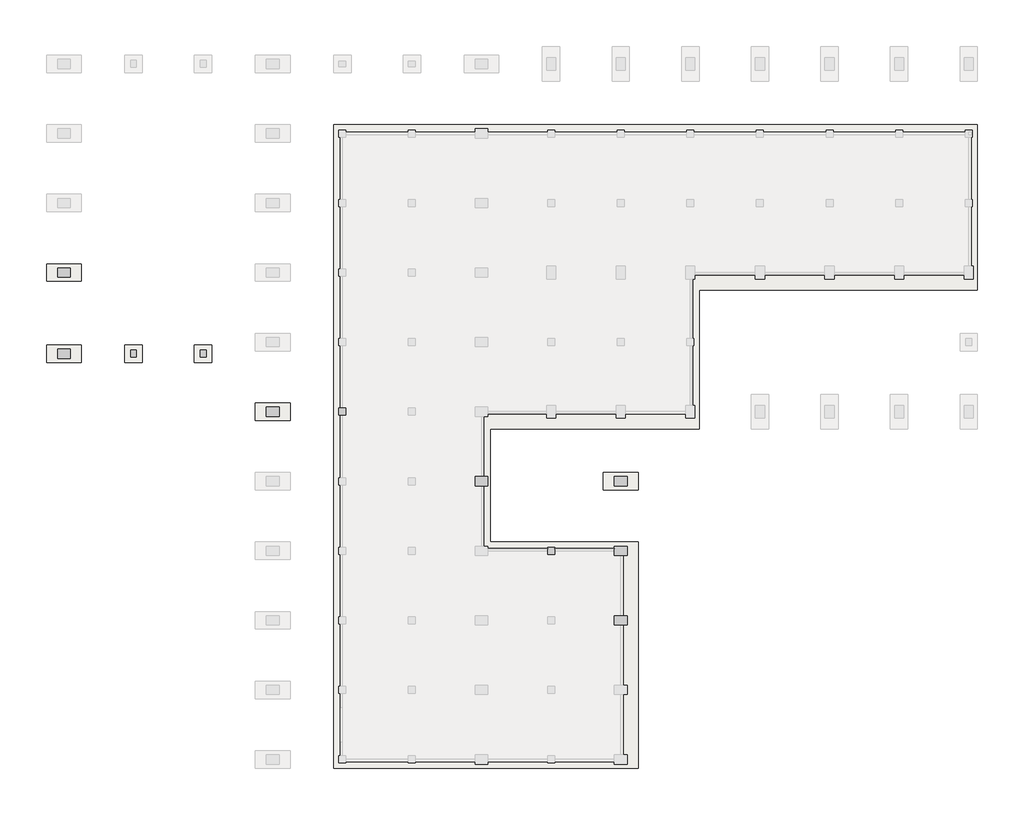
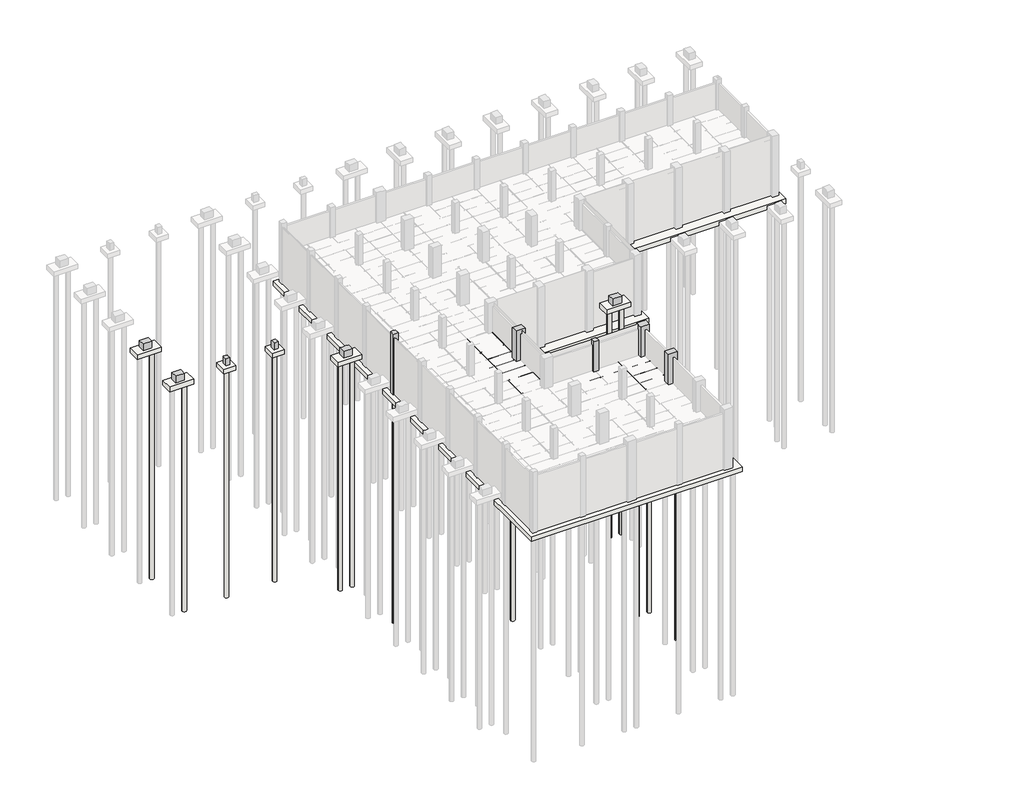
# Not in any storey, part 6 of 16: 20 slabs, 16 beams, 11 columns.
"""IFC4 building model written with IfcOpenShell, lengths in millimetres."""

from ifc_helpers import new_model, si_unit, point, frame, frame_2d, origin, place, context, project, spatial, polyline, circle_curve, trimmed, segment, composite_curve, outline, extrude, faceted_brep, element, save

model = new_model("IFC4")

# Units and contexts
model_context = context("Model", 3, world=origin())
ifc_project = project(units=[si_unit("LENGTHUNIT", "METRE", prefix="MILLI")], contexts=[model_context])

# Site, building
site = spatial("IfcSite", under=ifc_project)
building = spatial("IfcBuilding", under=site)

# Beams
placement = place(None, origin())
element("IfcBeam", 1, ObjectType="Steel Framing_C_KS : H_SB_AR_S02_C-150x75x6.5x10_J1", at=placement, inside=building, context=model_context, shape_type="SweptSolid", body=[
    extrude(outline(composite_curve([segment(polyline([(-43477.2, -3800.0381366), (-43477.2, -3950.0381366), (-43552.2, -3950.0381366)]), True, "CONTINUOUS"), segment(trimmed(circle_curve(frame_2d((-43542.2, -3950.0381366)), 10.0), [point((-43552.2, -3950.0381366))], [point((-43542.2, -3940.0381366))], False, "CARTESIAN"), True, "CONTINUOUS"), segment(polyline([(-43542.2, -3940.0381366), (-43483.7, -3930.7726469), (-43483.7, -3819.3036264), (-43542.2, -3810.0381366)]), True, "CONTINUOUS"), segment(trimmed(circle_curve(frame_2d((-43542.2, -3800.0381366)), 10.0), [point((-43542.2, -3810.0381366))], [point((-43552.2, -3800.0381366))], False, "CARTESIAN"), True, "CONTINUOUS"), segment(polyline([(-43552.2, -3800.0381366), (-43477.2, -3800.0381366)]), True, "CONTINUOUS")], self_intersect=False)), frame((39112.7, 0.0, 0.0), z_axis=(1.0, 0.0, 0.0), x_axis=(0.0, 1.0, 0.0)), (0.0, 0.0, 1.0), 2774.6),
])
element("IfcBeam", 2, ObjectType="Steel Framing_H_KS : H_SB_AR_S02_H-400x200x8x13_BSB1", at=placement, inside=building, context=model_context, shape_type="SweptSolid", body=[
    extrude(outline(composite_curve([segment(polyline([(-4187.0381366, 44900.0), (-4200.0381366, 44900.0), (-4200.0381366, 45100.0), (-4187.0381366, 45100.0), (-4187.0381366, 45020.0)]), True, "CONTINUOUS"), segment(trimmed(circle_curve(frame_2d((-4171.0381366, 45020.0)), 16.0), [point((-4187.0381366, 45020.0))], [point((-4171.0381366, 45004.0))], True, "CARTESIAN"), True, "CONTINUOUS"), segment(polyline([(-4171.0381366, 45004.0), (-3829.0381366, 45004.0)]), True, "CONTINUOUS"), segment(trimmed(circle_curve(frame_2d((-3829.0381366, 45020.0)), 16.0), [point((-3829.0381366, 45004.0))], [point((-3813.0381366, 45020.0))], True, "CARTESIAN"), True, "CONTINUOUS"), segment(polyline([(-3813.0381366, 45020.0), (-3813.0381366, 45100.0), (-3800.0381366, 45100.0), (-3800.0381366, 44900.0), (-3813.0381366, 44900.0), (-3813.0381366, 44980.0)]), True, "CONTINUOUS"), segment(trimmed(circle_curve(frame_2d((-3829.0381366, 44980.0)), 16.0), [point((-3813.0381366, 44980.0))], [point((-3829.0381366, 44996.0))], True, "CARTESIAN"), True, "CONTINUOUS"), segment(polyline([(-3829.0381366, 44996.0), (-4171.0381366, 44996.0)]), True, "CONTINUOUS"), segment(trimmed(circle_curve(frame_2d((-4171.0381366, 44980.0)), 16.0), [point((-4171.0381366, 44996.0))], [point((-4187.0381366, 44980.0))], True, "CARTESIAN"), True, "CONTINUOUS"), segment(polyline([(-4187.0381366, 44980.0), (-4187.0381366, 44900.0)]), True, "CONTINUOUS")], self_intersect=False)), frame((0.0, -47887.3, 0.0), z_axis=(0.0, 1.0, 0.0), x_axis=(0.0, 0.0, 1.0)), (0.0, 0.0, 1.0), 5887.3),
])
element("IfcBeam", 3, ObjectType="Steel Framing_C_KS : H_SB_AR_S02_C-150x75x6.5x10_J1", at=placement, inside=building, context=model_context, shape_type="SweptSolid", body=[
    extrude(outline(composite_curve([segment(polyline([(-43477.2, -3800.0381366), (-43477.2, -3950.0381366), (-43552.2, -3950.0381366)]), True, "CONTINUOUS"), segment(trimmed(circle_curve(frame_2d((-43542.2, -3950.0381366)), 10.0), [point((-43552.2, -3950.0381366))], [point((-43542.2, -3940.0381366))], False, "CARTESIAN"), True, "CONTINUOUS"), segment(polyline([(-43542.2, -3940.0381366), (-43483.7, -3930.7726469), (-43483.7, -3819.3036264), (-43542.2, -3810.0381366)]), True, "CONTINUOUS"), segment(trimmed(circle_curve(frame_2d((-43542.2, -3800.0381366)), 10.0), [point((-43542.2, -3810.0381366))], [point((-43552.2, -3800.0381366))], False, "CARTESIAN"), True, "CONTINUOUS"), segment(polyline([(-43552.2, -3800.0381366), (-43477.2, -3800.0381366)]), True, "CONTINUOUS")], self_intersect=False)), frame((42112.7, 0.0, 0.0), z_axis=(1.0, 0.0, 0.0), x_axis=(0.0, 1.0, 0.0)), (0.0, 0.0, 1.0), 2774.6),
])
element("IfcBeam", 4, ObjectType="Steel Framing_C_KS : H_SB_AR_S02_C-150x75x6.5x10_J1", at=placement, inside=building, context=model_context, shape_type="SweptSolid", body=[
    extrude(outline(composite_curve([segment(polyline([(-44977.2, -3800.0381366), (-44977.2, -3950.0381366), (-45052.2, -3950.0381366)]), True, "CONTINUOUS"), segment(trimmed(circle_curve(frame_2d((-45042.2, -3950.0381366)), 10.0), [point((-45052.2, -3950.0381366))], [point((-45042.2, -3940.0381366))], False, "CARTESIAN"), True, "CONTINUOUS"), segment(polyline([(-45042.2, -3940.0381366), (-44983.7, -3930.7726469), (-44983.7, -3819.3036264), (-45042.2, -3810.0381366)]), True, "CONTINUOUS"), segment(trimmed(circle_curve(frame_2d((-45042.2, -3800.0381366)), 10.0), [point((-45042.2, -3810.0381366))], [point((-45052.2, -3800.0381366))], False, "CARTESIAN"), True, "CONTINUOUS"), segment(polyline([(-45052.2, -3800.0381366), (-44977.2, -3800.0381366)]), True, "CONTINUOUS")], self_intersect=False)), frame((45112.7, 0.0, 0.0), z_axis=(1.0, 0.0, 0.0), x_axis=(0.0, 1.0, 0.0)), (0.0, 0.0, 1.0), 2887.3),
])
element("IfcBeam", 5, ObjectType="Steel Framing_C_KS : H_SB_AR_S02_C-150x75x6.5x10_J1", at=placement, inside=building, context=model_context, shape_type="SweptSolid", body=[
    extrude(outline(composite_curve([segment(polyline([(-46477.2, -3800.0381366), (-46477.2, -3950.0381366), (-46552.2, -3950.0381366)]), True, "CONTINUOUS"), segment(trimmed(circle_curve(frame_2d((-46542.2, -3950.0381366)), 10.0), [point((-46552.2, -3950.0381366))], [point((-46542.2, -3940.0381366))], False, "CARTESIAN"), True, "CONTINUOUS"), segment(polyline([(-46542.2, -3940.0381366), (-46483.7, -3930.7726469), (-46483.7, -3819.3036264), (-46542.2, -3810.0381366)]), True, "CONTINUOUS"), segment(trimmed(circle_curve(frame_2d((-46542.2, -3800.0381366)), 10.0), [point((-46542.2, -3810.0381366))], [point((-46552.2, -3800.0381366))], False, "CARTESIAN"), True, "CONTINUOUS"), segment(polyline([(-46552.2, -3800.0381366), (-46477.2, -3800.0381366)]), True, "CONTINUOUS")], self_intersect=False)), frame((45112.7, 0.0, 0.0), z_axis=(1.0, 0.0, 0.0), x_axis=(0.0, 1.0, 0.0)), (0.0, 0.0, 1.0), 2887.3),
])
element("IfcBeam", 6, ObjectType="Steel Framing_C_KS : H_SB_AR_S02_C-150x75x6.5x10_J1", at=placement, inside=building, context=model_context, shape_type="SweptSolid", body=[
    extrude(outline(composite_curve([segment(polyline([(-43477.2, -3800.0381366), (-43477.2, -3950.0381366), (-43552.2, -3950.0381366)]), True, "CONTINUOUS"), segment(trimmed(circle_curve(frame_2d((-43542.2, -3950.0381366)), 10.0), [point((-43552.2, -3950.0381366))], [point((-43542.2, -3940.0381366))], False, "CARTESIAN"), True, "CONTINUOUS"), segment(polyline([(-43542.2, -3940.0381366), (-43483.7, -3930.7726469), (-43483.7, -3819.3036264), (-43542.2, -3810.0381366)]), True, "CONTINUOUS"), segment(trimmed(circle_curve(frame_2d((-43542.2, -3800.0381366)), 10.0), [point((-43542.2, -3810.0381366))], [point((-43552.2, -3800.0381366))], False, "CARTESIAN"), True, "CONTINUOUS"), segment(polyline([(-43552.2, -3800.0381366), (-43477.2, -3800.0381366)]), True, "CONTINUOUS")], self_intersect=False)), frame((45112.7, 0.0, 0.0), z_axis=(1.0, 0.0, 0.0), x_axis=(0.0, 1.0, 0.0)), (0.0, 0.0, 1.0), 2887.3),
])
element("IfcBeam", 7, ObjectType="Steel Framing_C_KS : H_SB_AR_S02_C-150x75x6.5x10_J1", at=placement, inside=building, context=model_context, shape_type="SweptSolid", body=[
    extrude(outline(composite_curve([segment(polyline([(-31477.2, -3800.0381366), (-31477.2, -3950.0381366), (-31552.2, -3950.0381366)]), True, "CONTINUOUS"), segment(trimmed(circle_curve(frame_2d((-31542.2, -3950.0381366)), 10.0), [point((-31552.2, -3950.0381366))], [point((-31542.2, -3940.0381366))], False, "CARTESIAN"), True, "CONTINUOUS"), segment(polyline([(-31542.2, -3940.0381366), (-31483.7, -3930.7726469), (-31483.7, -3819.3036264), (-31542.2, -3810.0381366)]), True, "CONTINUOUS"), segment(trimmed(circle_curve(frame_2d((-31542.2, -3800.0381366)), 10.0), [point((-31542.2, -3810.0381366))], [point((-31552.2, -3800.0381366))], False, "CARTESIAN"), True, "CONTINUOUS"), segment(polyline([(-31552.2, -3800.0381366), (-31477.2, -3800.0381366)]), True, "CONTINUOUS")], self_intersect=False)), frame((24000.0, 0.0, 0.0), z_axis=(1.0, 0.0, 0.0), x_axis=(0.0, 1.0, 0.0)), (0.0, 0.0, 1.0), 2887.3),
])
element("IfcBeam", 8, ObjectType="Steel Framing_H_KS : H_SB_AR_S02_H-400x200x8x13_BSG1", at=placement, inside=building, context=model_context, shape_type="SweptSolid", body=[
    extrude(outline(composite_curve([segment(polyline([(-35900.0, -4187.0381366), (-35900.0, -4200.0381366), (-36100.0, -4200.0381366), (-36100.0, -4187.0381366), (-36020.0, -4187.0381366)]), True, "CONTINUOUS"), segment(trimmed(circle_curve(frame_2d((-36020.0, -4171.0381366)), 16.0), [point((-36020.0, -4187.0381366))], [point((-36004.0, -4171.0381366))], True, "CARTESIAN"), True, "CONTINUOUS"), segment(polyline([(-36004.0, -4171.0381366), (-36004.0, -3829.0381366)]), True, "CONTINUOUS"), segment(trimmed(circle_curve(frame_2d((-36020.0, -3829.0381366)), 16.0), [point((-36004.0, -3829.0381366))], [point((-36020.0, -3813.0381366))], True, "CARTESIAN"), True, "CONTINUOUS"), segment(polyline([(-36020.0, -3813.0381366), (-36100.0, -3813.0381366), (-36100.0, -3800.0381366), (-35900.0, -3800.0381366), (-35900.0, -3813.0381366), (-35980.0, -3813.0381366)]), True, "CONTINUOUS"), segment(trimmed(circle_curve(frame_2d((-35980.0, -3829.0381366)), 16.0), [point((-35980.0, -3813.0381366))], [point((-35996.0, -3829.0381366))], True, "CARTESIAN"), True, "CONTINUOUS"), segment(polyline([(-35996.0, -3829.0381366), (-35996.0, -4171.0381366)]), True, "CONTINUOUS"), segment(trimmed(circle_curve(frame_2d((-35980.0, -4171.0381366)), 16.0), [point((-35996.0, -4171.0381366))], [point((-35980.0, -4187.0381366))], True, "CARTESIAN"), True, "CONTINUOUS"), segment(polyline([(-35980.0, -4187.0381366), (-35900.0, -4187.0381366)]), True, "CONTINUOUS")], self_intersect=False)), frame((30312.7, 0.0, 0.0), z_axis=(1.0, 0.0, 0.0), x_axis=(0.0, 1.0, 0.0)), (0.0, 0.0, 1.0), 5124.6),
])
element("IfcBeam", 9, ObjectType="Steel Framing_H_KS : H_SB_AR_S02_H-400x200x8x13_BSG2", at=placement, inside=building, context=model_context, shape_type="SweptSolid", body=[
    extrude(outline(composite_curve([segment(polyline([(-4187.0381366, 35900.0), (-4200.0381366, 35900.0), (-4200.0381366, 36100.0), (-4187.0381366, 36100.0), (-4187.0381366, 36020.0)]), True, "CONTINUOUS"), segment(trimmed(circle_curve(frame_2d((-4171.0381366, 36020.0)), 16.0), [point((-4187.0381366, 36020.0))], [point((-4171.0381366, 36004.0))], True, "CARTESIAN"), True, "CONTINUOUS"), segment(polyline([(-4171.0381366, 36004.0), (-3829.0381366, 36004.0)]), True, "CONTINUOUS"), segment(trimmed(circle_curve(frame_2d((-3829.0381366, 36020.0)), 16.0), [point((-3829.0381366, 36004.0))], [point((-3813.0381366, 36020.0))], True, "CARTESIAN"), True, "CONTINUOUS"), segment(polyline([(-3813.0381366, 36020.0), (-3813.0381366, 36100.0), (-3800.0381366, 36100.0), (-3800.0381366, 35900.0), (-3813.0381366, 35900.0), (-3813.0381366, 35980.0)]), True, "CONTINUOUS"), segment(trimmed(circle_curve(frame_2d((-3829.0381366, 35980.0)), 16.0), [point((-3813.0381366, 35980.0))], [point((-3829.0381366, 35996.0))], True, "CARTESIAN"), True, "CONTINUOUS"), segment(polyline([(-3829.0381366, 35996.0), (-4171.0381366, 35996.0)]), True, "CONTINUOUS"), segment(trimmed(circle_curve(frame_2d((-4171.0381366, 35980.0)), 16.0), [point((-4171.0381366, 35996.0))], [point((-4187.0381366, 35980.0))], True, "CARTESIAN"), True, "CONTINUOUS"), segment(polyline([(-4187.0381366, 35980.0), (-4187.0381366, 35900.0)]), True, "CONTINUOUS")], self_intersect=False)), frame((0.0, -35587.3, 0.0), z_axis=(0.0, 1.0, 0.0), x_axis=(0.0, 0.0, 1.0)), (0.0, 0.0, 1.0), 5174.6),
])
element("IfcBeam", 10, ObjectType="Steel Framing_H_KS : H_SB_AR_S02_H-400x200x8x13_BSB1", at=placement, inside=building, context=model_context, shape_type="SweptSolid", body=[
    extrude(outline(composite_curve([segment(polyline([(-4187.0381366, 32900.0), (-4200.0381366, 32900.0), (-4200.0381366, 33100.0), (-4187.0381366, 33100.0), (-4187.0381366, 33020.0)]), True, "CONTINUOUS"), segment(trimmed(circle_curve(frame_2d((-4171.0381366, 33020.0)), 16.0), [point((-4187.0381366, 33020.0))], [point((-4171.0381366, 33004.0))], True, "CARTESIAN"), True, "CONTINUOUS"), segment(polyline([(-4171.0381366, 33004.0), (-3829.0381366, 33004.0)]), True, "CONTINUOUS"), segment(trimmed(circle_curve(frame_2d((-3829.0381366, 33020.0)), 16.0), [point((-3829.0381366, 33004.0))], [point((-3813.0381366, 33020.0))], True, "CARTESIAN"), True, "CONTINUOUS"), segment(polyline([(-3813.0381366, 33020.0), (-3813.0381366, 33100.0), (-3800.0381366, 33100.0), (-3800.0381366, 32900.0), (-3813.0381366, 32900.0), (-3813.0381366, 32980.0)]), True, "CONTINUOUS"), segment(trimmed(circle_curve(frame_2d((-3829.0381366, 32980.0)), 16.0), [point((-3813.0381366, 32980.0))], [point((-3829.0381366, 32996.0))], True, "CARTESIAN"), True, "CONTINUOUS"), segment(polyline([(-3829.0381366, 32996.0), (-4171.0381366, 32996.0)]), True, "CONTINUOUS"), segment(trimmed(circle_curve(frame_2d((-4171.0381366, 32980.0)), 16.0), [point((-4171.0381366, 32996.0))], [point((-4187.0381366, 32980.0))], True, "CARTESIAN"), True, "CONTINUOUS"), segment(polyline([(-4187.0381366, 32980.0), (-4187.0381366, 32900.0)]), True, "CONTINUOUS")], self_intersect=False)), frame((0.0, -35887.3, 0.0), z_axis=(0.0, 1.0, 0.0), x_axis=(0.0, 0.0, 1.0)), (0.0, 0.0, 1.0), 5774.6),
])
element("IfcBeam", 11, ObjectType="Steel Framing_C_KS : H_SB_AR_S02_C-150x75x6.5x10_J1", at=placement, inside=building, context=model_context, shape_type="SweptSolid", body=[
    extrude(outline(composite_curve([segment(polyline([(-32977.2, -3800.0381366), (-32977.2, -3950.0381366), (-33052.2, -3950.0381366)]), True, "CONTINUOUS"), segment(trimmed(circle_curve(frame_2d((-33042.2, -3950.0381366)), 10.0), [point((-33052.2, -3950.0381366))], [point((-33042.2, -3940.0381366))], False, "CARTESIAN"), True, "CONTINUOUS"), segment(polyline([(-33042.2, -3940.0381366), (-32983.7, -3930.7726469), (-32983.7, -3819.3036264), (-33042.2, -3810.0381366)]), True, "CONTINUOUS"), segment(trimmed(circle_curve(frame_2d((-33042.2, -3800.0381366)), 10.0), [point((-33042.2, -3810.0381366))], [point((-33052.2, -3800.0381366))], False, "CARTESIAN"), True, "CONTINUOUS"), segment(polyline([(-33052.2, -3800.0381366), (-32977.2, -3800.0381366)]), True, "CONTINUOUS")], self_intersect=False)), frame((33112.7, 0.0, 0.0), z_axis=(1.0, 0.0, 0.0), x_axis=(0.0, 1.0, 0.0)), (0.0, 0.0, 1.0), 2774.6),
])
element("IfcBeam", 12, ObjectType="Steel Framing_C_KS : H_SB_AR_S02_C-150x75x6.5x10_J1", at=placement, inside=building, context=model_context, shape_type="SweptSolid", body=[
    extrude(outline(composite_curve([segment(polyline([(-34477.2, -3800.0381366), (-34477.2, -3950.0381366), (-34552.2, -3950.0381366)]), True, "CONTINUOUS"), segment(trimmed(circle_curve(frame_2d((-34542.2, -3950.0381366)), 10.0), [point((-34552.2, -3950.0381366))], [point((-34542.2, -3940.0381366))], False, "CARTESIAN"), True, "CONTINUOUS"), segment(polyline([(-34542.2, -3940.0381366), (-34483.7, -3930.7726469), (-34483.7, -3819.3036264), (-34542.2, -3810.0381366)]), True, "CONTINUOUS"), segment(trimmed(circle_curve(frame_2d((-34542.2, -3800.0381366)), 10.0), [point((-34542.2, -3810.0381366))], [point((-34552.2, -3800.0381366))], False, "CARTESIAN"), True, "CONTINUOUS"), segment(polyline([(-34552.2, -3800.0381366), (-34477.2, -3800.0381366)]), True, "CONTINUOUS")], self_intersect=False)), frame((33112.7, 0.0, 0.0), z_axis=(1.0, 0.0, 0.0), x_axis=(0.0, 1.0, 0.0)), (0.0, 0.0, 1.0), 2774.6),
])
element("IfcBeam", 13, ObjectType="Steel Framing_H_KS : H_SB_AR_S02_H-400x200x8x13_BSG2", at=placement, inside=building, context=model_context, shape_type="SweptSolid", body=[
    extrude(outline(composite_curve([segment(polyline([(-4187.0381366, 35900.0), (-4200.0381366, 35900.0), (-4200.0381366, 36100.0), (-4187.0381366, 36100.0), (-4187.0381366, 36020.0)]), True, "CONTINUOUS"), segment(trimmed(circle_curve(frame_2d((-4171.0381366, 36020.0)), 16.0), [point((-4187.0381366, 36020.0))], [point((-4171.0381366, 36004.0))], True, "CARTESIAN"), True, "CONTINUOUS"), segment(polyline([(-4171.0381366, 36004.0), (-3829.0381366, 36004.0)]), True, "CONTINUOUS"), segment(trimmed(circle_curve(frame_2d((-3829.0381366, 36020.0)), 16.0), [point((-3829.0381366, 36004.0))], [point((-3813.0381366, 36020.0))], True, "CARTESIAN"), True, "CONTINUOUS"), segment(polyline([(-3813.0381366, 36020.0), (-3813.0381366, 36100.0), (-3800.0381366, 36100.0), (-3800.0381366, 35900.0), (-3813.0381366, 35900.0), (-3813.0381366, 35980.0)]), True, "CONTINUOUS"), segment(trimmed(circle_curve(frame_2d((-3829.0381366, 35980.0)), 16.0), [point((-3813.0381366, 35980.0))], [point((-3829.0381366, 35996.0))], True, "CARTESIAN"), True, "CONTINUOUS"), segment(polyline([(-3829.0381366, 35996.0), (-4171.0381366, 35996.0)]), True, "CONTINUOUS"), segment(trimmed(circle_curve(frame_2d((-4171.0381366, 35980.0)), 16.0), [point((-4171.0381366, 35996.0))], [point((-4187.0381366, 35980.0))], True, "CARTESIAN"), True, "CONTINUOUS"), segment(polyline([(-4187.0381366, 35980.0), (-4187.0381366, 35900.0)]), True, "CONTINUOUS")], self_intersect=False)), frame((0.0, -41587.3, 0.0), z_axis=(0.0, 1.0, 0.0), x_axis=(0.0, 0.0, 1.0)), (0.0, 0.0, 1.0), 5174.6),
])
element("IfcBeam", 14, ObjectType="Steel Framing_H_KS : H_SB_AR_S02_H-400x200x8x13_BSB1", at=placement, inside=building, context=model_context, shape_type="SweptSolid", body=[
    extrude(outline(composite_curve([segment(polyline([(-4187.0381366, 32900.0), (-4200.0381366, 32900.0), (-4200.0381366, 33100.0), (-4187.0381366, 33100.0), (-4187.0381366, 33020.0)]), True, "CONTINUOUS"), segment(trimmed(circle_curve(frame_2d((-4171.0381366, 33020.0)), 16.0), [point((-4187.0381366, 33020.0))], [point((-4171.0381366, 33004.0))], True, "CARTESIAN"), True, "CONTINUOUS"), segment(polyline([(-4171.0381366, 33004.0), (-3829.0381366, 33004.0)]), True, "CONTINUOUS"), segment(trimmed(circle_curve(frame_2d((-3829.0381366, 33020.0)), 16.0), [point((-3829.0381366, 33004.0))], [point((-3813.0381366, 33020.0))], True, "CARTESIAN"), True, "CONTINUOUS"), segment(polyline([(-3813.0381366, 33020.0), (-3813.0381366, 33100.0), (-3800.0381366, 33100.0), (-3800.0381366, 32900.0), (-3813.0381366, 32900.0), (-3813.0381366, 32980.0)]), True, "CONTINUOUS"), segment(trimmed(circle_curve(frame_2d((-3829.0381366, 32980.0)), 16.0), [point((-3813.0381366, 32980.0))], [point((-3829.0381366, 32996.0))], True, "CARTESIAN"), True, "CONTINUOUS"), segment(polyline([(-3829.0381366, 32996.0), (-4171.0381366, 32996.0)]), True, "CONTINUOUS"), segment(trimmed(circle_curve(frame_2d((-4171.0381366, 32980.0)), 16.0), [point((-4171.0381366, 32996.0))], [point((-4187.0381366, 32980.0))], True, "CARTESIAN"), True, "CONTINUOUS"), segment(polyline([(-4187.0381366, 32980.0), (-4187.0381366, 32900.0)]), True, "CONTINUOUS")], self_intersect=False)), frame((0.0, -41887.3, 0.0), z_axis=(0.0, 1.0, 0.0), x_axis=(0.0, 0.0, 1.0)), (0.0, 0.0, 1.0), 5774.6),
])
element("IfcBeam", 15, ObjectType="Steel Framing_C_KS : H_SB_AR_S02_C-150x75x6.5x10_J1", at=placement, inside=building, context=model_context, shape_type="SweptSolid", body=[
    extrude(outline(composite_curve([segment(polyline([(-38977.2, -3800.0381366), (-38977.2, -3950.0381366), (-39052.2, -3950.0381366)]), True, "CONTINUOUS"), segment(trimmed(circle_curve(frame_2d((-39042.2, -3950.0381366)), 10.0), [point((-39052.2, -3950.0381366))], [point((-39042.2, -3940.0381366))], False, "CARTESIAN"), True, "CONTINUOUS"), segment(polyline([(-39042.2, -3940.0381366), (-38983.7, -3930.7726469), (-38983.7, -3819.3036264), (-39042.2, -3810.0381366)]), True, "CONTINUOUS"), segment(trimmed(circle_curve(frame_2d((-39042.2, -3800.0381366)), 10.0), [point((-39042.2, -3810.0381366))], [point((-39052.2, -3800.0381366))], False, "CARTESIAN"), True, "CONTINUOUS"), segment(polyline([(-39052.2, -3800.0381366), (-38977.2, -3800.0381366)]), True, "CONTINUOUS")], self_intersect=False)), frame((33112.7, 0.0, 0.0), z_axis=(1.0, 0.0, 0.0), x_axis=(0.0, 1.0, 0.0)), (0.0, 0.0, 1.0), 2774.6),
])
element("IfcBeam", 16, ObjectType="Steel Framing_C_KS : H_SB_AR_S02_C-150x75x6.5x10_J1", at=placement, inside=building, context=model_context, shape_type="SweptSolid", body=[
    extrude(outline(composite_curve([segment(polyline([(-37477.2, -3800.0381366), (-37477.2, -3950.0381366), (-37552.2, -3950.0381366)]), True, "CONTINUOUS"), segment(trimmed(circle_curve(frame_2d((-37542.2, -3950.0381366)), 10.0), [point((-37552.2, -3950.0381366))], [point((-37542.2, -3940.0381366))], False, "CARTESIAN"), True, "CONTINUOUS"), segment(polyline([(-37542.2, -3940.0381366), (-37483.7, -3930.7726469), (-37483.7, -3819.3036264), (-37542.2, -3810.0381366)]), True, "CONTINUOUS"), segment(trimmed(circle_curve(frame_2d((-37542.2, -3800.0381366)), 10.0), [point((-37542.2, -3810.0381366))], [point((-37552.2, -3800.0381366))], False, "CARTESIAN"), True, "CONTINUOUS"), segment(polyline([(-37552.2, -3800.0381366), (-37477.2, -3800.0381366)]), True, "CONTINUOUS")], self_intersect=False)), frame((33112.7, 0.0, 0.0), z_axis=(1.0, 0.0, 0.0), x_axis=(0.0, 1.0, 0.0)), (0.0, 0.0, 1.0), 2774.6),
])

# Columns
element("IfcColumn", 17, ObjectType="RC_Column_Rectangular : H_SC_AR_S15_UG PED_Bit_800x1100_PD1", at=placement, inside=building, context=model_context, shape_type="Brep", body=[
    faceted_brep([(35450.0, -35600.0, -7800.0381366), (36000.0, -35600.0, -7800.0381366), (36200.0, -35600.0, -7800.0381366), (36550.0, -35600.0, -7800.0381366), (36550.0, -36400.0, -7800.0381366), (36200.0, -36400.0, -7800.0381366), (36000.0, -36400.0, -7800.0381366), (35450.0, -36400.0, -7800.0381366), (35450.0, -35600.0, 199.9618634), (35825.0, -35600.0, 199.9618634), (36175.0, -35600.0, 199.9618634), (36550.0, -35600.0, 199.9618634), (36550.0, -35600.0, -0.0381366), (35450.0, -35600.0, -3832.0381366), (35450.0, -35600.0, -3800.0381366), (35450.0, -35600.0, -0.0381366), (36550.0, -36400.0, 199.9618634), (36550.0, -36400.0, -0.0381366), (36175.0, -36400.0, 199.9618634), (35825.0, -36400.0, 199.9618634), (35450.0, -36400.0, 199.9618634), (35450.0, -36400.0, -0.0381366), (35450.0, -36400.0, -3800.0381366), (35450.0, -36400.0, -3832.0381366), (35450.0, -36175.0, 199.9618634), (35450.0, -35825.0, 199.9618634)], [[[0, 1, 2, 3, 4, 5, 6, 7]], [[8, 9, 10, 11, 12, 3, 2, 1, 0, 13, 14, 15]], [[11, 16, 17, 4, 3, 12]], [[16, 18, 19, 20, 21, 22, 23, 7, 6, 5, 4, 17]], [[20, 24, 25, 8, 15, 14, 13, 0, 7, 23, 22, 21]], [[8, 25, 24, 20, 19, 18, 16, 11, 10, 9]]]),
])
element("IfcColumn", 18, ObjectType="RC_Column_Rectangular : H_SC_AR_S15_UG PED_Bit_800x1100_PD1", at=placement, inside=building, context=model_context, shape_type="Brep", body=[
    faceted_brep([(47450.0, -47600.0, -7800.0381366), (48000.0, -47600.0, -7800.0381366), (48200.0, -47600.0, -7800.0381366), (48550.0, -47600.0, -7800.0381366), (48550.0, -48400.0, -7800.0381366), (48200.0, -48400.0, -7800.0381366), (48000.0, -48400.0, -7800.0381366), (47450.0, -48400.0, -7800.0381366), (47450.0, -47600.0, 199.9618634), (48000.0, -47600.0, 199.9618634), (48200.0, -47600.0, 199.9618634), (48550.0, -47600.0, 199.9618634), (47450.0, -47600.0, -3832.0381366), (47450.0, -47600.0, -3800.0381366), (47450.0, -47600.0, -0.0381366), (48550.0, -48400.0, 199.9618634), (48200.0, -48400.0, 199.9618634), (48000.0, -48400.0, 199.9618634), (47450.0, -48400.0, 199.9618634), (47450.0, -48400.0, -0.0381366), (47450.0, -48400.0, -3800.0381366), (47450.0, -48400.0, -3832.0381366), (47450.0, -48175.0, 199.9618634), (47450.0, -47825.0, 199.9618634)], [[[0, 1, 2, 3, 4, 5, 6, 7]], [[8, 9, 10, 11, 3, 2, 1, 0, 12, 13, 14]], [[11, 15, 4, 3]], [[15, 16, 17, 18, 19, 20, 21, 7, 6, 5, 4]], [[18, 22, 23, 8, 14, 13, 12, 0, 7, 21, 20, 19]], [[8, 23, 22, 18, 17, 16, 15, 11, 10, 9]]]),
])
element("IfcColumn", 19, ObjectType="RC_Column_Rectangular : H_SC_AR_S15_UG PED_Bit_800x1100_PD1", at=placement, inside=building, context=model_context, shape_type="Brep", body=[
    faceted_brep([(47450.0, -41600.0, -7800.0381366), (48550.0, -41600.0, -7800.0381366), (48550.0, -42400.0, -7800.0381366), (48200.0, -42400.0, -7800.0381366), (48000.0, -42400.0, -7800.0381366), (47450.0, -42400.0, -7800.0381366), (47450.0, -42000.0, -7800.0381366), (47450.0, -41800.0, -7800.0381366), (47450.0, -41600.0, 199.9618634), (47800.0, -41600.0, 199.9618634), (48200.0, -41600.0, 199.9618634), (48450.0, -41600.0, 199.9618634), (48550.0, -41600.0, 199.9618634), (47450.0, -41600.0, -0.0381366), (48550.0, -42400.0, 199.9618634), (48200.0, -42400.0, 199.9618634), (48000.0, -42400.0, 199.9618634), (47450.0, -42400.0, 199.9618634), (47450.0, -42400.0, -0.0381366), (47450.0, -42400.0, -3800.0381366), (47450.0, -42400.0, -3832.0381366), (47450.0, -42175.0, 199.9618634), (47450.0, -41825.0, 199.9618634), (47450.0, -41800.0, 199.9618634)], [[[0, 1, 2, 3, 4, 5, 6, 7]], [[8, 9, 10, 11, 12, 1, 0, 13]], [[12, 14, 2, 1]], [[14, 15, 16, 17, 18, 19, 20, 5, 4, 3, 2]], [[17, 21, 22, 23, 8, 13, 0, 7, 6, 5, 20, 19, 18]], [[8, 23, 22, 21, 17, 16, 15, 14, 12, 11, 10, 9]]]),
])
element("IfcColumn", 20, ObjectType="RC_Column_Rectangular : H_SC_AR_S15_UG PED_Bit_800x1100_PD1", at=placement, inside=building, context=model_context, shape_type="Brep", body=[
    faceted_brep([(-550.0, -17600.0, -700.0381366), (550.0, -17600.0, -700.0381366), (550.0, -18400.0, -700.0381366), (-550.0, -18400.0, -700.0381366), (-550.0, -17600.0, 199.9618634), (-200.0, -17600.0, 199.9618634), (200.0, -17600.0, 199.9618634), (550.0, -17600.0, 199.9618634), (550.0, -17600.0, -0.0381366), (550.0, -18400.0, 199.9618634), (550.0, -18400.0, -0.0381366), (200.0, -18400.0, 199.9618634), (-200.0, -18400.0, 199.9618634), (-550.0, -18400.0, 199.9618634)], [[[0, 1, 2, 3]], [[4, 5, 6, 7, 8, 1, 0]], [[7, 9, 10, 2, 1, 8]], [[9, 11, 12, 13, 3, 2, 10]], [[13, 4, 0, 3]], [[4, 13, 12, 11, 9, 7, 6, 5]]]),
])
element("IfcColumn", 21, ObjectType="RC_Column_Rectangular : H_SC_AR_S15_UG PED_Bit_800x1100_PD1", at=placement, inside=building, context=model_context, shape_type="Brep", body=[
    faceted_brep([(-550.0, -24600.0, -700.0381366), (550.0, -24600.0, -700.0381366), (550.0, -25400.0, -700.0381366), (-550.0, -25400.0, -700.0381366), (-550.0, -24600.0, 199.9618634), (200.0, -24600.0, 199.9618634), (550.0, -24600.0, 199.9618634), (550.0, -24600.0, -0.0381366), (550.0, -24800.0, 199.9618634), (550.0, -25400.0, 199.9618634), (-550.0, -25400.0, 199.9618634)], [[[0, 1, 2, 3]], [[4, 5, 6, 7, 1, 0]], [[6, 8, 9, 2, 1, 7]], [[9, 10, 3, 2]], [[10, 4, 0, 3]], [[4, 10, 9, 8, 6, 5]]]),
])
element("IfcColumn", 22, ObjectType="RC_Column_Rectangular : H_SC_AR_S15_UG PED_Bit_800x1100_PD1", at=placement, inside=building, context=model_context, shape_type="Brep", body=[
    faceted_brep([(17450.0, -29600.0, -700.0381366), (18550.0, -29600.0, -700.0381366), (18550.0, -30400.0, -700.0381366), (17450.0, -30400.0, -700.0381366), (17450.0, -29600.0, 199.9618634), (17800.0, -29600.0, 199.9618634), (18200.0, -29600.0, 199.9618634), (18550.0, -29600.0, 199.9618634), (18550.0, -29600.0, -0.0381366), (18550.0, -30400.0, 199.9618634), (18550.0, -30400.0, -0.0381366), (18200.0, -30400.0, 199.9618634), (17800.0, -30400.0, 199.9618634), (17450.0, -30400.0, 199.9618634)], [[[0, 1, 2, 3]], [[4, 5, 6, 7, 8, 1, 0]], [[7, 9, 10, 2, 1, 8]], [[9, 11, 12, 13, 3, 2, 10]], [[13, 4, 0, 3]], [[4, 13, 12, 11, 9, 7, 6, 5]]]),
])
element("IfcColumn", 23, ObjectType="RC_Column_Rectangular : H_SC_AR_S15_UG PED_Bit_800x1100_PD1", at=placement, inside=building, context=model_context, shape_type="Brep", body=[
    faceted_brep([(47450.0, -35600.0, -700.0381366), (48550.0, -35600.0, -700.0381366), (48550.0, -36400.0, -700.0381366), (47450.0, -36400.0, -700.0381366), (47450.0, -35600.0, 199.9618634), (47800.0, -35600.0, 199.9618634), (48200.0, -35600.0, 199.9618634), (48450.0, -35600.0, 199.9618634), (48550.0, -35600.0, 199.9618634), (47450.0, -35600.0, -0.0381366), (48550.0, -36400.0, 199.9618634), (48450.0, -36400.0, 199.9618634), (48200.0, -36400.0, 199.9618634), (47800.0, -36400.0, 199.9618634), (47450.0, -36400.0, 199.9618634), (47450.0, -36400.0, -0.0381366)], [[[0, 1, 2, 3]], [[4, 5, 6, 7, 8, 1, 0, 9]], [[8, 10, 2, 1]], [[10, 11, 12, 13, 14, 15, 3, 2]], [[14, 4, 9, 0, 3, 15]], [[4, 14, 13, 12, 11, 10, 8, 7, 6, 5]]]),
])
element("IfcColumn", 24, ObjectType="RC_Column_Rectangular : H_SC_AR_S15_UG PED_Bit_600x600_BC1", at=placement, inside=building, context=model_context, shape_type="Brep", body=[
    faceted_brep([(24300.0, -29700.0, -7800.0381366), (24300.0, -30300.0, -7800.0381366), (24000.0, -30300.0, -7800.0381366), (23800.0, -30300.0, -7800.0381366), (23700.0, -30300.0, -7800.0381366), (23700.0, -29700.0, -7800.0381366), (23800.0, -29700.0, -7800.0381366), (24000.0, -29700.0, -7800.0381366), (24300.0, -29700.0, 199.9618634), (24300.0, -29825.0, 199.9618634), (24300.0, -30175.0, 199.9618634), (24300.0, -30300.0, 199.9618634), (24300.0, -30300.0, -0.0381366), (24300.0, -30300.0, -3800.0381366), (24300.0, -30300.0, -3832.0381366), (24300.0, -29700.0, -3832.0381366), (24300.0, -29700.0, -3800.0381366), (24300.0, -29700.0, -0.0381366), (24000.0, -30300.0, 199.9618634), (23700.0, -30300.0, 199.9618634), (23700.0, -30300.0, -0.0381366), (23700.0, -29700.0, 199.9618634), (23700.0, -29700.0, -0.0381366), (24000.0, -29700.0, 199.9618634)], [[[0, 1, 2, 3, 4, 5, 6, 7]], [[8, 9, 10, 11, 12, 13, 14, 1, 0, 15, 16, 17]], [[11, 18, 19, 20, 4, 3, 2, 1, 14, 13, 12]], [[19, 21, 22, 5, 4, 20]], [[21, 23, 8, 17, 16, 15, 0, 7, 6, 5, 22]], [[8, 23, 21, 19, 18, 11, 10, 9]]]),
])
element("IfcColumn", 25, ObjectType="RC_Column_Rectangular : H_SC_AR_S15_UG PED_Bit_600x600_BC1", at=placement, inside=building, context=model_context, shape_type="Brep", body=[
    faceted_brep([(42300.0, -41700.0, -7200.0381366), (42300.0, -41800.0, -7200.0381366), (42300.0, -42000.0, -7200.0381366), (42300.0, -42300.0, -7200.0381366), (41700.0, -42300.0, -7200.0381366), (41700.0, -42000.0, -7200.0381366), (41700.0, -41800.0, -7200.0381366), (41700.0, -41700.0, -7200.0381366), (42300.0, -41700.0, 199.9618634), (42300.0, -41800.0, 199.9618634), (42300.0, -41825.0, 199.9618634), (42300.0, -42175.0, 199.9618634), (42300.0, -42300.0, 199.9618634), (42300.0, -42300.0, -0.0381366), (42300.0, -42300.0, -3800.0381366), (42300.0, -42300.0, -3832.0381366), (42300.0, -41700.0, -0.0381366), (42175.0, -42300.0, 199.9618634), (41825.0, -42300.0, 199.9618634), (41700.0, -42300.0, 199.9618634), (41700.0, -42300.0, -0.0381366), (41700.0, -42300.0, -3800.0381366), (41700.0, -42300.0, -3832.0381366), (41700.0, -42175.0, 199.9618634), (41700.0, -41825.0, 199.9618634), (41700.0, -41800.0, 199.9618634), (41700.0, -41700.0, 199.9618634), (41700.0, -41700.0, -0.0381366)], [[[0, 1, 2, 3, 4, 5, 6, 7]], [[8, 9, 10, 11, 12, 13, 14, 15, 3, 2, 1, 0, 16]], [[12, 17, 18, 19, 20, 21, 22, 4, 3, 15, 14, 13]], [[19, 23, 24, 25, 26, 27, 7, 6, 5, 4, 22, 21, 20]], [[26, 8, 16, 0, 7, 27]], [[8, 26, 25, 24, 23, 19, 18, 17, 12, 11, 10, 9]]]),
])
element("IfcColumn", 26, ObjectType="RC_Column_Rectangular : H_SC_AR_S15_UG PED_Bit_500x600_PD2", at=placement, inside=building, context=model_context, shape_type="Brep", body=[
    faceted_brep([(5750.0, -25300.0, -700.0381366), (5750.0, -24700.0, -700.0381366), (6250.0, -24700.0, -700.0381366), (6250.0, -25300.0, -700.0381366), (5750.0, -25300.0, 199.9618634), (5750.0, -25200.0, 199.9618634), (5750.0, -24800.0, 199.9618634), (5750.0, -24700.0, 199.9618634), (5750.0, -24700.0, -0.0381366), (6250.0, -24700.0, 199.9618634), (6250.0, -24700.0, -0.0381366), (6250.0, -24800.0, 199.9618634), (6250.0, -25200.0, 199.9618634), (6250.0, -25300.0, 199.9618634)], [[[0, 1, 2, 3]], [[4, 5, 6, 7, 8, 1, 0]], [[7, 9, 10, 2, 1, 8]], [[9, 11, 12, 13, 3, 2, 10]], [[13, 4, 0, 3]], [[4, 13, 12, 11, 9, 7, 6, 5]]]),
])
element("IfcColumn", 27, ObjectType="RC_Column_Rectangular : H_SC_AR_S15_UG PED_Bit_500x600_PD2", at=placement, inside=building, context=model_context, shape_type="Brep", body=[
    faceted_brep([(11750.0, -25300.0, -700.0381366), (11750.0, -24700.0, -700.0381366), (12250.0, -24700.0, -700.0381366), (12250.0, -25300.0, -700.0381366), (11750.0, -25300.0, 199.9618634), (11750.0, -25200.0, 199.9618634), (11750.0, -24800.0, 199.9618634), (11750.0, -24700.0, 199.9618634), (11750.0, -24700.0, -0.0381366), (12250.0, -24700.0, 199.9618634), (12250.0, -24700.0, -0.0381366), (12250.0, -24800.0, 199.9618634), (12250.0, -25200.0, 199.9618634), (12250.0, -25300.0, 199.9618634)], [[[0, 1, 2, 3]], [[4, 5, 6, 7, 8, 1, 0]], [[7, 9, 10, 2, 1, 8]], [[9, 11, 12, 13, 3, 2, 10]], [[13, 4, 0, 3]], [[4, 13, 12, 11, 9, 7, 6, 5]]]),
])

# Slabs
element("IfcSlab", 28, ObjectType="H_SF_AR_S18_MAT_Bitumen_T600_MF1", at=placement, inside=building, context=model_context, shape_type="Brep", body=[
    faceted_brep([(78750.0, -5250.0, -8400.0381366), (78750.0, -19500.0, -8400.0381366), (54750.0, -19500.0, -8400.0381366), (54750.0, -31500.0, -8400.0381366), (36750.0, -31500.0, -8400.0381366), (36750.0, -35750.0, -8400.0381366), (36750.0, -36250.0, -8400.0381366), (36750.0, -41250.0, -8400.0381366), (49500.0, -41250.0, -8400.0381366), (49500.0, -60750.0, -8400.0381366), (23250.0, -60750.0, -8400.0381366), (23250.0, -5250.0, -8400.0381366), (78750.0, -5250.0, -7800.0381366), (23250.0, -5250.0, -7800.0381366), (23250.0, -60750.0, -7800.0381366), (49500.0, -60750.0, -7800.0381366), (49500.0, -41250.0, -7800.0381366), (36750.0, -41250.0, -7800.0381366), (36750.0, -36250.0, -7800.0381366), (36750.0, -35750.0, -7800.0381366), (36750.0, -31500.0, -7800.0381366), (54750.0, -31500.0, -7800.0381366), (54750.0, -19500.0, -7800.0381366), (78750.0, -19500.0, -7800.0381366)], [[[0, 1, 2, 3, 4, 5, 6, 7, 8, 9, 10, 11]], [[12, 13, 14, 15, 16, 17, 18, 19, 20, 21, 22, 23]], [[1, 0, 12, 23]], [[2, 1, 23, 22]], [[3, 2, 22, 21]], [[4, 3, 21, 20]], [[7, 6, 5, 4, 20, 19, 18, 17]], [[8, 7, 17, 16]], [[9, 8, 16, 15]], [[10, 9, 15, 14]], [[11, 10, 14, 13]], [[0, 11, 13, 12]]]),
])
element("IfcSlab", 29, ObjectType="Foundation Rectangular (Non-Pile) : H_SF_AR_S18_Shallow Fdn_Bitumen_1500x3000xT600_F1", at=placement, inside=building, context=model_context, shape_type="SweptSolid", body=[
    extrude(outline(polyline([(1500.0, -18750.0), (-1500.0, -18750.0), (-1500.0, -17250.0), (1500.0, -17250.0), (1500.0, -18750.0)])), frame((0.0, 0.0, -1300.0381366), z_axis=(0.0, 0.0, 1.0), x_axis=(1.0, 0.0, 0.0)), (0.0, 0.0, 1.0), 600.0),
])
element("IfcSlab", 30, ObjectType="Foundation Rectangular (Non-Pile) : H_SF_AR_S18_Shallow Fdn_Bitumen_1500x3000xT600_F1", at=placement, inside=building, context=model_context, shape_type="SweptSolid", body=[
    extrude(outline(polyline([(1500.0, -25750.0), (-1500.0, -25750.0), (-1500.0, -24250.0), (1500.0, -24250.0), (1500.0, -25750.0)])), frame((0.0, 0.0, -1300.0381366), z_axis=(0.0, 0.0, 1.0), x_axis=(1.0, 0.0, 0.0)), (0.0, 0.0, 1.0), 600.0),
])
element("IfcSlab", 31, ObjectType="Foundation Rectangular (Non-Pile) : H_SF_AR_S18_Shallow Fdn_Bitumen_1500x3000xT600_F1", at=placement, inside=building, context=model_context, shape_type="SweptSolid", body=[
    extrude(outline(polyline([(19500.0, -30750.0), (16500.0, -30750.0), (16500.0, -29250.0), (19500.0, -29250.0), (19500.0, -30750.0)])), frame((0.0, 0.0, -1300.0381366), z_axis=(0.0, 0.0, 1.0), x_axis=(1.0, 0.0, 0.0)), (0.0, 0.0, 1.0), 600.0),
])
element("IfcSlab", 32, ObjectType="Foundation Rectangular (Non-Pile) : H_SF_AR_S18_Shallow Fdn_Bitumen_1500x3000xT600_F1", at=placement, inside=building, context=model_context, shape_type="SweptSolid", body=[
    extrude(outline(polyline([(49500.0, -36750.0), (46500.0, -36750.0), (46500.0, -35250.0), (49500.0, -35250.0), (49500.0, -36750.0)])), frame((0.0, 0.0, -1300.0381366), z_axis=(0.0, 0.0, 1.0), x_axis=(1.0, 0.0, 0.0)), (0.0, 0.0, 1.0), 600.0),
])
element("IfcSlab", 33, ObjectType="Foundation Rectangular (Non-Pile) : H_SF_AR_S18_Shallow Fdn_Bitumen_1500x1500xT600_F2", at=placement, inside=building, context=model_context, shape_type="SweptSolid", body=[
    extrude(outline(polyline([(6750.0, -25750.0), (5250.0, -25750.0), (5250.0, -24250.0), (6750.0, -24250.0), (6750.0, -25750.0)])), frame((0.0, 0.0, -1300.0381366), z_axis=(0.0, 0.0, 1.0), x_axis=(1.0, 0.0, 0.0)), (0.0, 0.0, 1.0), 600.0),
])
element("IfcSlab", 34, ObjectType="Foundation Rectangular (Non-Pile) : H_SF_AR_S18_Shallow Fdn_Bitumen_1500x1500xT600_F2", at=placement, inside=building, context=model_context, shape_type="SweptSolid", body=[
    extrude(outline(polyline([(12750.0, -25750.0), (11250.0, -25750.0), (11250.0, -24250.0), (12750.0, -24250.0), (12750.0, -25750.0)])), frame((0.0, 0.0, -1300.0381366), z_axis=(0.0, 0.0, 1.0), x_axis=(1.0, 0.0, 0.0)), (0.0, 0.0, 1.0), 600.0),
])
element("IfcSlab", 35, ObjectType="PILE : H_SF_AR_S19_PHC Pile_Pre-boring_D500_L30", at=placement, inside=building, context=model_context, shape_type="SweptSolid", body=[
    extrude(outline(composite_curve([segment(trimmed(circle_curve(frame_2d((17250.0, -30000.0)), 250.0), [point((17000.0, -30000.0))], [point((17500.0, -30000.0))], False, "CARTESIAN"), True, "CONTINUOUS"), segment(trimmed(circle_curve(frame_2d((17250.0, -30000.0)), 250.0), [point((17500.0, -30000.0))], [point((17000.0, -30000.0))], False, "CARTESIAN"), True, "CONTINUOUS")], self_intersect=False)), frame((0.0, 0.0, -31300.0381366), z_axis=(0.0, 0.0, 1.0), x_axis=(1.0, 0.0, 0.0)), (0.0, 0.0, 1.0), 30000.0),
])
element("IfcSlab", 36, ObjectType="PILE : H_SF_AR_S19_PHC Pile_Pre-boring_D500_L30", at=placement, inside=building, context=model_context, shape_type="SweptSolid", body=[
    extrude(outline(composite_curve([segment(trimmed(circle_curve(frame_2d((18750.0, -30000.0)), 250.0), [point((18500.0, -30000.0))], [point((19000.0, -30000.0))], False, "CARTESIAN"), True, "CONTINUOUS"), segment(trimmed(circle_curve(frame_2d((18750.0, -30000.0)), 250.0), [point((19000.0, -30000.0))], [point((18500.0, -30000.0))], False, "CARTESIAN"), True, "CONTINUOUS")], self_intersect=False)), frame((0.0, 0.0, -31300.0381366), z_axis=(0.0, 0.0, 1.0), x_axis=(1.0, 0.0, 0.0)), (0.0, 0.0, 1.0), 30000.0),
])
element("IfcSlab", 37, ObjectType="PILE : H_SF_AR_S19_PHC Pile_Pre-boring_D500_L30", at=placement, inside=building, context=model_context, shape_type="SweptSolid", body=[
    extrude(outline(composite_curve([segment(trimmed(circle_curve(frame_2d((750.0, -25000.0)), 250.0), [point((500.0, -25000.0))], [point((1000.0, -25000.0))], False, "CARTESIAN"), True, "CONTINUOUS"), segment(trimmed(circle_curve(frame_2d((750.0, -25000.0)), 250.0), [point((1000.0, -25000.0))], [point((500.0, -25000.0))], False, "CARTESIAN"), True, "CONTINUOUS")], self_intersect=False)), frame((0.0, 0.0, -31300.0381366), z_axis=(0.0, 0.0, 1.0), x_axis=(1.0, 0.0, 0.0)), (0.0, 0.0, 1.0), 30000.0),
])
element("IfcSlab", 38, ObjectType="PILE : H_SF_AR_S19_PHC Pile_Pre-boring_D500_L30", at=placement, inside=building, context=model_context, shape_type="SweptSolid", body=[
    extrude(outline(composite_curve([segment(trimmed(circle_curve(frame_2d((750.0, -18000.0)), 250.0), [point((500.0, -18000.0))], [point((1000.0, -18000.0))], False, "CARTESIAN"), True, "CONTINUOUS"), segment(trimmed(circle_curve(frame_2d((750.0, -18000.0)), 250.0), [point((1000.0, -18000.0))], [point((500.0, -18000.0))], False, "CARTESIAN"), True, "CONTINUOUS")], self_intersect=False)), frame((0.0, 0.0, -31300.0381366), z_axis=(0.0, 0.0, 1.0), x_axis=(1.0, 0.0, 0.0)), (0.0, 0.0, 1.0), 30000.0),
])
element("IfcSlab", 39, ObjectType="PILE : H_SF_AR_S19_PHC Pile_Pre-boring_D500_L30", at=placement, inside=building, context=model_context, shape_type="SweptSolid", body=[
    extrude(outline(composite_curve([segment(trimmed(circle_curve(frame_2d((47250.0, -36000.0)), 250.0), [point((47000.0, -36000.0))], [point((47500.0, -36000.0))], False, "CARTESIAN"), True, "CONTINUOUS"), segment(trimmed(circle_curve(frame_2d((47250.0, -36000.0)), 250.0), [point((47500.0, -36000.0))], [point((47000.0, -36000.0))], False, "CARTESIAN"), True, "CONTINUOUS")], self_intersect=False)), frame((0.0, 0.0, -31300.0381366), z_axis=(0.0, 0.0, 1.0), x_axis=(1.0, 0.0, 0.0)), (0.0, 0.0, 1.0), 30000.0),
])
element("IfcSlab", 40, ObjectType="PILE : H_SF_AR_S19_PHC Pile_Pre-boring_D500_L30", at=placement, inside=building, context=model_context, shape_type="SweptSolid", body=[
    extrude(outline(composite_curve([segment(trimmed(circle_curve(frame_2d((48750.0, -36000.0)), 250.0), [point((48500.0, -36000.0))], [point((49000.0, -36000.0))], False, "CARTESIAN"), True, "CONTINUOUS"), segment(trimmed(circle_curve(frame_2d((48750.0, -36000.0)), 250.0), [point((49000.0, -36000.0))], [point((48500.0, -36000.0))], False, "CARTESIAN"), True, "CONTINUOUS")], self_intersect=False)), frame((0.0, 0.0, -31300.0381366), z_axis=(0.0, 0.0, 1.0), x_axis=(1.0, 0.0, 0.0)), (0.0, 0.0, 1.0), 30000.0),
])
element("IfcSlab", 41, ObjectType="PILE : H_SF_AR_S19_PHC Pile_Pre-boring_D500_L30", at=placement, inside=building, context=model_context, shape_type="SweptSolid", body=[
    extrude(outline(composite_curve([segment(trimmed(circle_curve(frame_2d((6000.0, -25000.0)), 250.0), [point((5750.0, -25000.0))], [point((6250.0, -25000.0))], False, "CARTESIAN"), True, "CONTINUOUS"), segment(trimmed(circle_curve(frame_2d((6000.0, -25000.0)), 250.0), [point((6250.0, -25000.0))], [point((5750.0, -25000.0))], False, "CARTESIAN"), True, "CONTINUOUS")], self_intersect=False)), frame((0.0, 0.0, -31300.0381366), z_axis=(0.0, 0.0, 1.0), x_axis=(1.0, 0.0, 0.0)), (0.0, 0.0, 1.0), 30000.0),
])
element("IfcSlab", 42, ObjectType="PILE : H_SF_AR_S19_PHC Pile_Pre-boring_D500_L30", at=placement, inside=building, context=model_context, shape_type="SweptSolid", body=[
    extrude(outline(composite_curve([segment(trimmed(circle_curve(frame_2d((12000.0, -25000.0)), 250.0), [point((11750.0, -25000.0))], [point((12250.0, -25000.0))], False, "CARTESIAN"), True, "CONTINUOUS"), segment(trimmed(circle_curve(frame_2d((12000.0, -25000.0)), 250.0), [point((12250.0, -25000.0))], [point((11750.0, -25000.0))], False, "CARTESIAN"), True, "CONTINUOUS")], self_intersect=False)), frame((0.0, 0.0, -31300.0381366), z_axis=(0.0, 0.0, 1.0), x_axis=(1.0, 0.0, 0.0)), (0.0, 0.0, 1.0), 30000.0),
])
element("IfcSlab", 43, ObjectType="PILE : H_SF_AR_S19_PHC Pile_Pre-boring_D500_L30", at=placement, inside=building, context=model_context, shape_type="SweptSolid", body=[
    extrude(outline(composite_curve([segment(trimmed(circle_curve(frame_2d((48750.0, -48000.0)), 250.0), [point((48500.0, -48000.0))], [point((49000.0, -48000.0))], False, "CARTESIAN"), True, "CONTINUOUS"), segment(trimmed(circle_curve(frame_2d((48750.0, -48000.0)), 250.0), [point((49000.0, -48000.0))], [point((48500.0, -48000.0))], False, "CARTESIAN"), True, "CONTINUOUS")], self_intersect=False)), frame((0.0, 0.0, -37950.0381366), z_axis=(0.0, 0.0, 1.0), x_axis=(1.0, 0.0, 0.0)), (0.0, 0.0, 1.0), 29550.0),
])
element("IfcSlab", 44, ObjectType="PILE : H_SF_AR_S19_PHC Pile_Pre-boring_D500_L30", at=placement, inside=building, context=model_context, shape_type="SweptSolid", body=[
    extrude(outline(composite_curve([segment(trimmed(circle_curve(frame_2d((47250.0, -42000.0)), 250.0), [point((47000.0, -42000.0))], [point((47500.0, -42000.0))], False, "CARTESIAN"), True, "CONTINUOUS"), segment(trimmed(circle_curve(frame_2d((47250.0, -42000.0)), 250.0), [point((47500.0, -42000.0))], [point((47000.0, -42000.0))], False, "CARTESIAN"), True, "CONTINUOUS")], self_intersect=False)), frame((0.0, 0.0, -37950.0381366), z_axis=(0.0, 0.0, 1.0), x_axis=(1.0, 0.0, 0.0)), (0.0, 0.0, 1.0), 29550.0),
])
element("IfcSlab", 45, ObjectType="PILE : H_SF_AR_S19_PHC Pile_Pre-boring_D500_L30", at=placement, inside=building, context=model_context, shape_type="SweptSolid", body=[
    extrude(outline(composite_curve([segment(trimmed(circle_curve(frame_2d((48750.0, -42000.0)), 250.0), [point((48500.0, -42000.0))], [point((49000.0, -42000.0))], False, "CARTESIAN"), True, "CONTINUOUS"), segment(trimmed(circle_curve(frame_2d((48750.0, -42000.0)), 250.0), [point((49000.0, -42000.0))], [point((48500.0, -42000.0))], False, "CARTESIAN"), True, "CONTINUOUS")], self_intersect=False)), frame((0.0, 0.0, -37950.0381366), z_axis=(0.0, 0.0, 1.0), x_axis=(1.0, 0.0, 0.0)), (0.0, 0.0, 1.0), 29550.0),
])
element("IfcSlab", 46, ObjectType="PILE : H_SF_AR_S19_PHC Pile_Pre-boring_D500_L30", at=placement, inside=building, context=model_context, shape_type="SweptSolid", body=[
    extrude(outline(composite_curve([segment(trimmed(circle_curve(frame_2d((35250.0, -36000.0)), 250.0), [point((35000.0, -36000.0))], [point((35500.0, -36000.0))], False, "CARTESIAN"), True, "CONTINUOUS"), segment(trimmed(circle_curve(frame_2d((35250.0, -36000.0)), 250.0), [point((35500.0, -36000.0))], [point((35000.0, -36000.0))], False, "CARTESIAN"), True, "CONTINUOUS")], self_intersect=False)), frame((0.0, 0.0, -37950.0381366), z_axis=(0.0, 0.0, 1.0), x_axis=(1.0, 0.0, 0.0)), (0.0, 0.0, 1.0), 29550.0),
])
element("IfcSlab", 47, ObjectType="PILE : H_SF_AR_S19_PHC Pile_Pre-boring_D500_L30", at=placement, inside=building, context=model_context, shape_type="SweptSolid", body=[
    extrude(outline(composite_curve([segment(trimmed(circle_curve(frame_2d((24000.0, -30000.0)), 250.0), [point((23750.0, -30000.0))], [point((24250.0, -30000.0))], False, "CARTESIAN"), True, "CONTINUOUS"), segment(trimmed(circle_curve(frame_2d((24000.0, -30000.0)), 250.0), [point((24250.0, -30000.0))], [point((23750.0, -30000.0))], False, "CARTESIAN"), True, "CONTINUOUS")], self_intersect=False)), frame((0.0, 0.0, -37950.0381366), z_axis=(0.0, 0.0, 1.0), x_axis=(1.0, 0.0, 0.0)), (0.0, 0.0, 1.0), 29550.0),
])

save(model, "model.ifc")

# Revit data of these elements
# Type "Steel Framing_C_KS : H_SB_AR_S02_C-150x75x6.5x10_J1"
#   Type Mark = "J1"
#   H_SectionID = "C-150x75x6.5x10"
#   Assembly Code = "B10"
#   H_Ratio for Additional Steel Plate = 0.2
#   Perimeter = 0.51 m²/m
#   Nominal Weight = 18.60 kgf/m
#   Length [instance default] = 1000 mm
#   bf = 75 mm
#   d = 150 mm
#   tf = 10 mm
#   tw = 6.5 mm
#   x = 22.8 mm
#   A = 0.002371 m²
#   Structural Material [instance default] = Steel, 45-345
# Type "Steel Framing_H_KS : H_SB_AR_S02_H-400x200x8x13_BSB1"
#   Type Comments = "MAIN"
#   Type Mark = "BSB1"
#   H_SectionID = "H-400x200x8x13"
#   H_Ratio for Additional Steel Plate = 0.2
#   Width = 20.0 cm
#   Web Thickness = 0.8 cm
#   Web Fillet = 1.6 cm
#   Warping Constant = 649000.0 cm⁶
#   Torsional Moment of Inertia = 35.8981 cm⁴
#   Section Area = 84.12 cm²
#   Plastic Modulus weak axis = 268.0 cm³
#   Plastic Modulus strong axis = 1330.0 cm³
#   Perimeter = 1.56 m²/m
#   Nominal Weight = 66.00 kgf/m
#   Moment of Inertia weak axis = 1740.00 cm⁴
#   Moment of Inertia strong axis = 23700.00 cm⁴
#   Height = 40.0 cm
#   Flange Thickness = 1.3 cm
#   Elastic Modulus weak axis = 174.0 cm³
#   Elastic Modulus strong axis = 1190.0 cm³
#   Centroid Vertical = 20.0 cm
#   Centroid Horizontal = 10.0 cm
#   Bolt Spacing = 8.89 cm
#   Length [instance default] = 1500 mm
#   Structural Material [instance default] = Steel, 45-345
#   Section Name Key = ""
#   Assembly Code = ""
# Type "Steel Framing_H_KS : H_SB_AR_S02_H-400x200x8x13_BSG1"
#   Type Comments = "MAIN"
#   Type Mark = "BSG1"
#   H_SectionID = "H-400x200x8x13"
#   H_Ratio for Additional Steel Plate = 0.2
#   Width = 20.0 cm
#   Web Thickness = 0.8 cm
#   Web Fillet = 1.6 cm
#   Warping Constant = 649000.0 cm⁶
#   Torsional Moment of Inertia = 35.8981 cm⁴
#   Section Area = 84.12 cm²
#   Plastic Modulus weak axis = 268.0 cm³
#   Plastic Modulus strong axis = 1330.0 cm³
#   Perimeter = 1.56 m²/m
#   Nominal Weight = 66.00 kgf/m
#   Moment of Inertia weak axis = 1740.00 cm⁴
#   Moment of Inertia strong axis = 23700.00 cm⁴
#   Height = 40.0 cm
#   Flange Thickness = 1.3 cm
#   Elastic Modulus weak axis = 174.0 cm³
#   Elastic Modulus strong axis = 1190.0 cm³
#   Centroid Vertical = 20.0 cm
#   Centroid Horizontal = 10.0 cm
#   Bolt Spacing = 8.89 cm
#   Length [instance default] = 1500 mm
#   Structural Material [instance default] = Steel, 45-345
#   Section Name Key = ""
#   Assembly Code = ""
# Type "Steel Framing_H_KS : H_SB_AR_S02_H-400x200x8x13_BSG2"
#   Type Comments = "MAIN"
#   Type Mark = "BSG2"
#   H_SectionID = "H-400x200x8x13"
#   H_Ratio for Additional Steel Plate = 0.2
#   Width = 20.0 cm
#   Web Thickness = 0.8 cm
#   Web Fillet = 1.6 cm
#   Warping Constant = 649000.0 cm⁶
#   Torsional Moment of Inertia = 35.8981 cm⁴
#   Section Area = 84.12 cm²
#   Plastic Modulus weak axis = 268.0 cm³
#   Plastic Modulus strong axis = 1330.0 cm³
#   Perimeter = 1.56 m²/m
#   Nominal Weight = 66.00 kgf/m
#   Moment of Inertia weak axis = 1740.00 cm⁴
#   Moment of Inertia strong axis = 23700.00 cm⁴
#   Height = 40.0 cm
#   Flange Thickness = 1.3 cm
#   Elastic Modulus weak axis = 174.0 cm³
#   Elastic Modulus strong axis = 1190.0 cm³
#   Centroid Vertical = 20.0 cm
#   Centroid Horizontal = 10.0 cm
#   Bolt Spacing = 8.89 cm
#   Length [instance default] = 1500 mm
#   Structural Material [instance default] = Steel, 45-345
#   Section Name Key = ""
#   Assembly Code = ""
# Type "RC_Column_Rectangular : H_SC_AR_S15_UG PED_Bit_800x1100_PD1"
#   Type Mark = "PD1"
#   Type Comments = "UG"
#   H_SectionID = "600 x 900"
#   H_Rebar Ratio = 0.3
#   Width = 800 mm
#   Depth = 1100 mm
#   hec_material3 [instance default] = none
#   hec_material2 [instance default] = none
#   hec_material1 [instance default] = none
#   Structural Material [instance default] = none
#   Description = (empty or 0)
# Type "RC_Column_Rectangular : H_SC_AR_S15_UG PED_Bit_600x600_BC1"
#   Type Mark = "BC1"
#   Type Comments = "UG"
#   H_SectionID = "600 x 600"
#   H_Rebar Ratio = 0.3
#   Width = 600 mm
#   Depth = 600 mm
#   hec_material3 [instance default] = none
#   hec_material2 [instance default] = none
#   hec_material1 [instance default] = none
#   Structural Material [instance default] = none
#   Description = (empty or 0)
# Type "RC_Column_Rectangular : H_SC_AR_S15_UG PED_Bit_500x600_PD2"
#   Type Mark = "PD2"
#   Type Comments = "UG"
#   H_SectionID = "600 x 900"
#   H_Rebar Ratio = 0.3
#   Width = 500 mm
#   Depth = 600 mm
#   hec_material3 [instance default] = none
#   hec_material2 [instance default] = none
#   hec_material1 [instance default] = none
#   Structural Material [instance default] = none
#   Description = (empty or 0)
# Type "H_SF_AR_S18_MAT_Bitumen_T600_MF1"
#   Type Comments = "MASS"
#   Type Mark = "MF1"
#   H_Rebar Ratio = 0.12
#   Layers, outside or top first: 600 mm "00_Concrete_Reinf. Conc." (function 1)
# Type "Foundation Rectangular (Non-Pile) : H_SF_AR_S18_Shallow Fdn_Bitumen_1500x3000xT600_F1"
#   Type Comments = "UG"
#   Type Mark = "F1"
#   Top bar = "D25@300"
#   Description = "UG Shallow Foundation"
#   Bottom bar = "D20@300"
#   H_Rebar Ratio = 0.12
#   Width = 1500 mm
#   Length = 3000 mm
#   Foundation Thickness = 600 mm
#   Structural Material [instance default] = none
#   Assembly Code = ""
# Type "Foundation Rectangular (Non-Pile) : H_SF_AR_S18_Shallow Fdn_Bitumen_1500x1500xT600_F2"
#   Type Comments = "UG"
#   Type Mark = "F2"
#   Top bar = "D25@300"
#   Description = "UG Shallow Foundation"
#   Bottom bar = "D20@300"
#   H_Rebar Ratio = 0.12
#   Width = 1500 mm
#   Length = 1500 mm
#   Foundation Thickness = 600 mm
#   Structural Material [instance default] = none
#   Assembly Code = ""
# Type "PILE : H_SF_AR_S19_PHC Pile_Pre-boring_D500_L30"
#   Assembly Code = "A1020120"
#   반지름 = 250 mm
#   최소 내포 = 150 mm
#   Diameter = 500 mm
#   Depth = 30000 mm
#   Structural Material [instance default] = none
# Elements 1, 3, 4, 5, 6, 7, 11, 12, 15, 16 (IfcBeam, "Steel Framing_C_KS : H_SB_AR_S02_C-150x75x6.5x10_J1")
#   Structural Material = Steel, 45-345
#   Phase Created = New Construction
